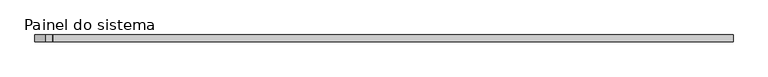
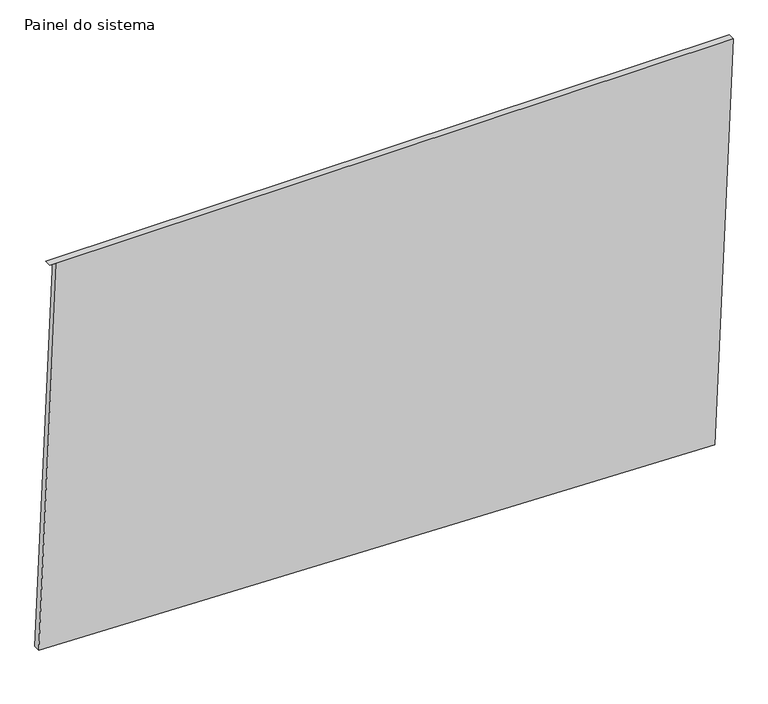
"""IFC4 building model written with IfcOpenShell, lengths in millimetres: plate geometry, Painel do sistema : Envidraçado."""

import ifcopenshell
import ifcopenshell.guid

model = None  # the IFC model being written
_history = None  # IfcOwnerHistory: only IFC2X3 demands one
_inside = {}  # id of a spatial element -> (the spatial element, [elements in it])
_under = {}  # id of a project, library or spatial element -> (it, [spatial elements below it])
_declared = {}  # id of a project -> (the project, [libraries it declares])
_typed = {}  # id of a type object -> (the type object, [elements of that type])
_made_of = {}  # id of a material, layer set ... -> (it, [elements and type objects made of it])


def new_model(schema):
    """Start an empty IFC model of exactly this schema.

    Asked for "IFC4X3", IfcOpenShell would pick the latest addendum, in which some entities
    have other attributes; the version numbers below select the first issue.
    IFC2X3 requires an IfcOwnerHistory on every rooted entity: one is made here for all.
    """
    global model, _history
    if schema == "IFC4X3":
        model = ifcopenshell.file(schema_version=(4, 3, 0, 0))
    else:
        model = ifcopenshell.file(schema=schema)
    _inside.clear()
    _under.clear()
    _declared.clear()
    _typed.clear()
    _made_of.clear()
    _history = None
    if model.schema == "IFC2X3":
        org = make("IfcOrganization", Name="unknown")
        user = make(
            "IfcPersonAndOrganization",
            ThePerson=make("IfcPerson", FamilyName="unknown"),
            TheOrganization=org,
        )
        app = make(
            "IfcApplication",
            ApplicationDeveloper=org,
            Version="unknown",
            ApplicationFullName="unknown",
            ApplicationIdentifier="unknown",
        )
        _history = make(
            "IfcOwnerHistory",
            OwningUser=user,
            OwningApplication=app,
            ChangeAction="ADDED",
            CreationDate=0,
        )
    return model


def make(cls, **values):
    """One entity of the class cls with the attributes given. An attribute that is None is left unset."""
    return model.create_entity(
        cls, **{name: value for name, value in values.items() if value is not None}
    )


def rooted(cls, **values):
    """An entity with a GlobalId (a new one), such as an element, a storey or a relation."""
    return make(cls, GlobalId=ifcopenshell.guid.new(), OwnerHistory=_history, **values)


def si_unit(unit_type, name, prefix=None):
    """IfcSIUnit, for example si_unit("LENGTHUNIT", "METRE", prefix="MILLI")."""
    return make("IfcSIUnit", UnitType=unit_type, Prefix=prefix, Name=name)


def assignment(units):
    """IfcUnitAssignment: the units of a project."""
    return None if units is None else make("IfcUnitAssignment", Units=units)


def point(xyz):
    """IfcCartesianPoint."""
    return None if xyz is None else make("IfcCartesianPoint", Coordinates=xyz)


def direction(xyz):
    """IfcDirection."""
    return None if xyz is None else make("IfcDirection", DirectionRatios=xyz)


def frame(location, z_axis=None, x_axis=None):
    """IfcAxis2Placement3D, a coordinate frame: its origin and axes. An axis left out is left unset."""
    return make(
        "IfcAxis2Placement3D",
        Location=point(location),
        Axis=direction(z_axis),
        RefDirection=direction(x_axis),
    )


def origin():
    """The frame at (0, 0, 0) with its axes left unset."""
    return frame((0.0, 0.0, 0.0))


def place(relative_to, where):
    """IfcLocalPlacement: puts the frame where relative to a parent placement (None: the world)."""
    return make(
        "IfcLocalPlacement", PlacementRelTo=relative_to, RelativePlacement=where
    )


def context(
    kind, dimensions, precision=None, world=None, true_north=None, identifier=None
):
    """IfcGeometricRepresentationContext, for example the 3D "Model" context."""
    return make(
        "IfcGeometricRepresentationContext",
        ContextIdentifier=identifier,
        ContextType=kind,
        CoordinateSpaceDimension=dimensions,
        Precision=precision,
        WorldCoordinateSystem=world,
        TrueNorth=true_north,
    )


def project(units=None, contexts=None):
    """IfcProject with its units and contexts."""
    return rooted(
        "IfcProject",
        Name="project",
        RepresentationContexts=contexts,
        UnitsInContext=assignment(units),
    )


def spatial(cls, under=None, at=None, **own):
    """A site, building, storey or space (cls), placed at a placement, below another one or the project."""
    s = rooted(cls, ObjectPlacement=at, **own)
    if under is not None:
        _under.setdefault(under.id(), (under, []))[1].append(s)
    return s


def polyline(points):
    """IfcPolyline through the points."""
    return make("IfcPolyline", Points=[point(p) for p in points])


def outline(outer, holes=None, kind="AREA"):
    """IfcArbitraryClosedProfileDef: a profile drawn as a closed curve; with holes, ...WithVoids."""
    if holes is None:
        return make("IfcArbitraryClosedProfileDef", ProfileType=kind, OuterCurve=outer)
    return make(
        "IfcArbitraryProfileDefWithVoids",
        ProfileType=kind,
        OuterCurve=outer,
        InnerCurves=holes,
    )


def extrude(swept, where, along, depth):
    """IfcExtrudedAreaSolid: the profile swept, set in the frame where, extruded along a direction by depth."""
    return make(
        "IfcExtrudedAreaSolid",
        SweptArea=swept,
        Position=where,
        ExtrudedDirection=direction(along),
        Depth=depth,
    )


def shape(context_of_items, identifier, shape_type, items):
    """IfcShapeRepresentation: the items that make up one representation, for example the "Body"."""
    return make(
        "IfcShapeRepresentation",
        ContextOfItems=context_of_items,
        RepresentationIdentifier=identifier,
        RepresentationType=shape_type,
        Items=items,
    )


def source(mapping_origin, context_of_items, identifier, shape_type, items):
    """IfcRepresentationMap: a shape defined once, which mapped items show again and again."""
    return make(
        "IfcRepresentationMap",
        MappingOrigin=mapping_origin,
        MappedRepresentation=shape(context_of_items, identifier, shape_type, items),
    )


def transform(
    local_origin,
    x_axis=None,
    y_axis=None,
    z_axis=None,
    scale=None,
    scale2=None,
    scale3=None,
    uniform=True,
):
    """IfcCartesianTransformationOperator3D, or its non-uniform kind. x_axis, y_axis, z_axis: its Axis1, 2, 3."""
    if uniform:
        return make(
            "IfcCartesianTransformationOperator3D",
            Axis1=direction(x_axis),
            Axis2=direction(y_axis),
            LocalOrigin=point(local_origin),
            Scale=scale,
            Axis3=direction(z_axis),
        )
    return make(
        "IfcCartesianTransformationOperator3DnonUniform",
        Axis1=direction(x_axis),
        Axis2=direction(y_axis),
        LocalOrigin=point(local_origin),
        Scale=scale,
        Axis3=direction(z_axis),
        Scale2=scale2,
        Scale3=scale3,
    )


def mapped(mapping_source, mapping_target):
    """IfcMappedItem: shows the shape of a source again, moved by a transform."""
    return make(
        "IfcMappedItem", MappingSource=mapping_source, MappingTarget=mapping_target
    )


def made_of(thing, what):
    """Note that an element or type object is made of a material, layer set ...; save() writes the relation."""
    if what is not None:
        _made_of.setdefault(what.id(), (what, []))[1].append(thing)
    return thing


def element(
    cls,
    number,
    at=None,
    inside=None,
    cuts=None,
    type_object=None,
    material=None,
    context=None,
    identifier="Body",
    shape_type=None,
    held_by="IfcProductDefinitionShape",
    body=None,
    shapes=None,
    **own,
):
    """One element of the class cls, such as IfcWall. Its Tag is "e" and its number.

    at: its placement. inside: the storey or other place that contains it. cuts: it is an
    opening in that element (IfcRelVoidsElement). A single representation is given by context,
    identifier, shape_type and body (its items); several are given by shapes. held_by: the class
    of the entity that holds the representations. save() writes the other relations.
    """
    e = rooted(cls, Tag="e%d" % number, ObjectPlacement=at, **own)
    if body is not None:
        shapes = [shape(context, identifier, shape_type, body)]
    if shapes is not None:
        e.Representation = make(held_by, Representations=shapes)
    if inside is not None:
        _inside.setdefault(inside.id(), (inside, []))[1].append(e)
    if cuts is not None:
        rooted(
            "IfcRelVoidsElement", RelatingBuildingElement=cuts, RelatedOpeningElement=e
        )
    if type_object is not None:
        _typed.setdefault(type_object.id(), (type_object, []))[1].append(e)
    return made_of(e, material)


def aggregate(whole, parts):
    """IfcRelAggregates: a whole, such as a stair, and the parts it consists of."""
    return rooted("IfcRelAggregates", RelatingObject=whole, RelatedObjects=parts)


def save(model, path):
    """Write the relations noted so far, then the file.

    IfcRelAggregates (storeys below a building ...), IfcRelContainedInSpatialStructure (elements
    in a storey), IfcRelDefinesByType, IfcRelAssociatesMaterial and IfcRelDeclares: one each for
    every whole, place, type object, material and project.
    """
    for whole, parts in _under.values():
        aggregate(whole, parts)
    for where, things in _inside.values():
        rooted(
            "IfcRelContainedInSpatialStructure",
            RelatedElements=things,
            RelatingStructure=where,
        )
    for kind, things in _typed.values():
        rooted("IfcRelDefinesByType", RelatedObjects=things, RelatingType=kind)
    for what, things in _made_of.values():
        rooted("IfcRelAssociatesMaterial", RelatedObjects=things, RelatingMaterial=what)
    for by, libraries in _declared.values():
        rooted("IfcRelDeclares", RelatingContext=by, RelatedDefinitions=libraries)
    model.write(path)


def painel_do_sistema_d9afe38d(model_context):
    return source(origin(), model_context, "Body", "SweptSolid", [
        extrude(outline(polyline([(72.8211161, -1295.6050124), (0.0, 1226.2580641), (1578.3869252, 1295.6050124), (1578.3869252, -1254.481601), (1577.2896005, -1229.5056951), (72.8211161, -1295.6050124)])), frame((0.0, 24.5, 0.0), z_axis=(0.0, 1.0, 0.0), x_axis=(0.0, 0.0, 1.0)), (0.0, 0.0, 1.0), 25.0),
    ])


if __name__ == "__main__":
    model = new_model("IFC4")
    model_context = context("Model", 3, world=origin())
    ifc_project = project(units=[si_unit("LENGTHUNIT", "METRE", prefix="MILLI")], contexts=[model_context])
    site = spatial("IfcSite", under=ifc_project)
    building = spatial("IfcBuilding", under=site)
    placement = place(None, origin())
    painel_do_sistema_shape = painel_do_sistema_d9afe38d(model_context)
    element("IfcPlate", 1, ObjectType="Painel do sistema : Envidraçado", at=placement, inside=building, context=model_context, shape_type="MappedRepresentation", body=[
        mapped(painel_do_sistema_shape, transform((0.0, 0.0, 0.0), x_axis=(1.0, 0.0, 0.0), y_axis=(0.0, 1.0, 0.0), z_axis=(0.0, 0.0, 1.0))),
    ])
    save(model, "model.ifc")

# Revit data of these elements
# Type "Painel do sistema : Envidraçado"
#   Construction Type Id = "GSP4R"
#   Analytic Construction = "Vidraça única Pilkington 1/8 pol"
#   Visual Light Transmittance = 0.9
#   Solar Heat Gain Coefficient = 0.86
#   Heat Transfer Coefficient (U) = 6.7069 W/(m²·K)
# Element 1 (IfcPlate, "Painel do sistema : Envidraçado")
#   Materials on its faces: "Vidro"
# Materials
#   "Vidro": class "Vidro", colour RGB 0 128 192, transparency 0.9, Description = "Vidro de sílica", Cost = 0
